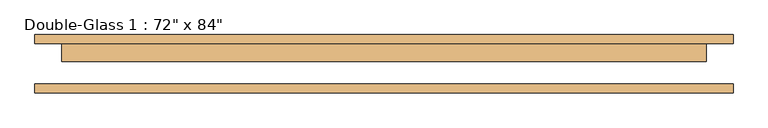
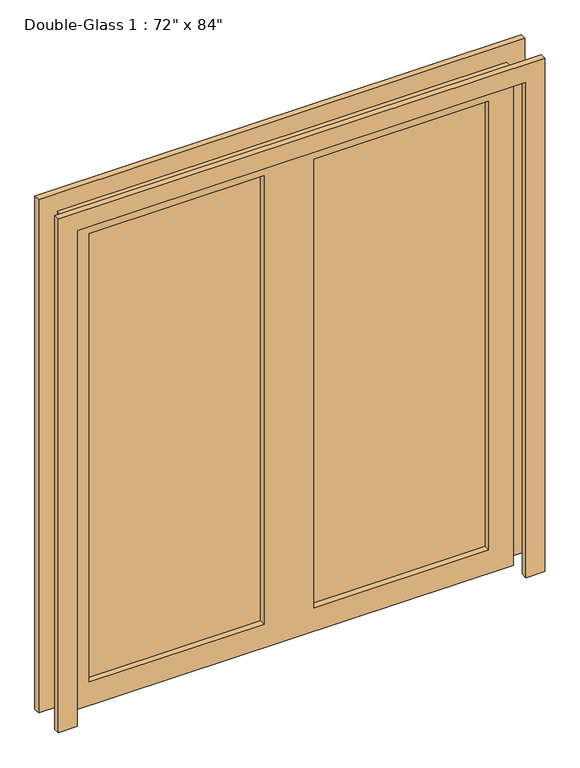
"""IFC4 building model written with IfcOpenShell, lengths in millimetres: door geometry."""

from ifc_helpers import new_model, si_unit, frame, origin, place, context, project, spatial, polyline, outline, extrude, source, transform, mapped, element, save


def door_1b837e8a(model_context):
    return source(origin(), model_context, "Body", "SweptSolid", [
        extrude(outline(polyline([(0.0, 990.6), (2209.8, 990.6), (2209.8, -990.6), (0.0, -990.6), (0.0, -914.4), (2133.6, -914.4), (2133.6, 914.4), (0.0, 914.4), (0.0, 990.6)])), frame((0.0, -80.16875, 0.0), z_axis=(0.0, 1.0, 0.0), x_axis=(0.0, 0.0, 1.0)), (0.0, 0.0, 1.0), 25.4),
        extrude(outline(polyline([(2133.6, 914.4), (0.0, 914.4), (0.0, 990.6), (2209.8, 990.6), (2209.8, -990.6), (0.0, -990.6), (0.0, -914.4), (2133.6, -914.4), (2133.6, 914.4)])), frame((0.0, 59.53125, 0.0), z_axis=(0.0, 1.0, 0.0), x_axis=(0.0, 0.0, 1.0)), (0.0, 0.0, 1.0), 25.4),
        extrude(outline(polyline([(812.8, 34.13125), (101.6, 34.13125), (101.6, 41.275), (812.8, 41.275), (812.8, 34.13125)])), frame((0.0, 0.0, 101.6), z_axis=(0.0, 0.0, 1.0), x_axis=(1.0, 0.0, 0.0)), (0.0, 0.0, 1.0), 1930.4),
        extrude(outline(polyline([(-101.6, 34.13125), (-812.8, 34.13125), (-812.8, 41.275), (-101.6, 41.275), (-101.6, 34.13125)])), frame((0.0, 0.0, 101.6), z_axis=(0.0, 0.0, 1.0), x_axis=(1.0, 0.0, 0.0)), (0.0, 0.0, 1.0), 1930.4),
        extrude(outline(polyline([(2133.6, 914.4), (2133.6, -914.4), (0.0, -914.4), (0.0, 914.4), (2133.6, 914.4)]), holes=[polyline([(2032.0, -101.6), (101.6, -101.6), (101.6, -812.8), (2032.0, -812.8), (2032.0, -101.6)]), polyline([(2032.0, 812.8), (101.6, 812.8), (101.6, 101.6), (2032.0, 101.6), (2032.0, 812.8)])]), frame((0.0, 8.73125, 0.0), z_axis=(0.0, 1.0, 0.0), x_axis=(0.0, 0.0, 1.0)), (0.0, 0.0, 1.0), 50.8),
    ])


if __name__ == "__main__":
    model = new_model("IFC4")
    model_context = context("Model", 3, world=origin())
    ifc_project = project(units=[si_unit("LENGTHUNIT", "METRE", prefix="MILLI")], contexts=[model_context])
    site = spatial("IfcSite", under=ifc_project)
    building = spatial("IfcBuilding", under=site)
    placement = place(None, origin())
    door_shape = door_1b837e8a(model_context)
    element("IfcDoor", 1, ObjectType="Double-Glass 1 : 72\" x 84\"", at=placement, inside=building, context=model_context, shape_type="MappedRepresentation", body=[
        mapped(door_shape, transform((0.0, 0.0, 0.0), x_axis=(1.0, 0.0, 0.0), y_axis=(0.0, 1.0, 0.0), z_axis=(0.0, 0.0, 1.0))),
    ])
    save(model, "model.ifc")

# Revit data of these elements
# Type "Double-Glass 1 : 72\" x 84\""
#   Type Mark = "34"
#   Assembly Code = "C1020"
#   Thickness = 0' - 2"
#   Height = 7' - 0"
#   Rail Width - Base = 0' - 4"
#   Rail Width - Top = 0' - 4"
#   Stile Width - Hinge = 0' - 4"
#   Stile Width - Latch = 0' - 4"
#   Trim Projection = 0' - 1"
#   Trim Width = 0' - 3"
#   Width = 6' - 0"
#   Function = 0
#   Door Material = Door - Panel
#   Frame Material = Door - Frame
#   Wall Closure = (empty or 0)
# Element 1 (IfcDoor, "Double-Glass 1 : 72\" x 84\"")
#   Materials on its faces: "Door - Frame", "Door - Panel", "Glass"
# Materials
#   "Door - Panel": class "Wood", colour RGB 230 193 158, transparency 0, Cost = 0
#   "Door - Frame": class "Paint", colour RGB 113 0 0, transparency 0, Cost = 0
#   "Glass": class "Glass", colour RGB 0 128 192, transparency 0.75, Cost = 0
